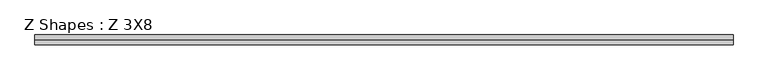
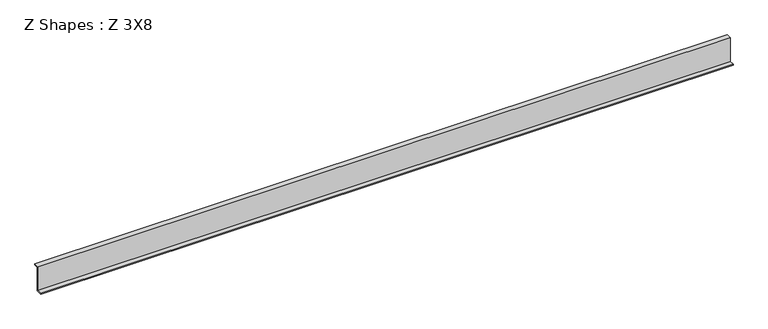
"""IFC4 building model written with IfcOpenShell, lengths in millimetres: beam geometry, Z Shapes : Z 3X8."""

from ifc_helpers import new_model, si_unit, frame, origin, place, context, project, spatial, polyline, outline, extrude, source, transform, mapped, element, save


def z_shapes_z_3x8_3d6c6c97(model_context):
    return source(origin(), model_context, "Body", "SweptSolid", [
        extrude(outline(polyline([(57.2805719, 92.452825), (27.1991352, 92.452825), (27.1991352, -98.809175), (-18.9194281, -98.809175), (-18.9194281, -92.459175), (19.1805719, -92.459175), (19.1805719, 102.104825), (57.2805719, 102.104825), (57.2805719, 92.452825)])), frame((-2667.0, 0.0, 0.0), z_axis=(1.0, 0.0, 0.0), x_axis=(0.0, 1.0, 0.0)), (0.0, 0.0, 1.0), 5334.0),
    ])


if __name__ == "__main__":
    model = new_model("IFC4")
    model_context = context("Model", 3, world=origin())
    ifc_project = project(units=[si_unit("LENGTHUNIT", "METRE", prefix="MILLI")], contexts=[model_context])
    site = spatial("IfcSite", under=ifc_project)
    building = spatial("IfcBuilding", under=site)
    placement = place(None, origin())
    z_shapes_z_3x8_shape = z_shapes_z_3x8_3d6c6c97(model_context)
    element("IfcBeam", 1, ObjectType="Z Shapes : Z 3X8", at=placement, inside=building, context=model_context, shape_type="MappedRepresentation", body=[
        mapped(z_shapes_z_3x8_shape, transform((0.0, 0.0, 0.0), x_axis=(1.0, 0.0, 0.0), y_axis=(0.0, 1.0, 0.0), z_axis=(0.0, 0.0, 1.0))),
    ])
    save(model, "model.ifc")

# Revit data of these elements
# Type "Z Shapes : Z 3X8"
#   Section Name Key = "W12x26"
#   Assembly Code = "B10"
#   Width = 76.2 mm
#   Web Thickness = 5.842 mm
#   Web Fillet = 7.62 mm
#   Warping Constant = 163001.3 cm⁶
#   Torsional Moment of Inertia = 12.4869 cm⁴
#   Section Area = 7.65 in²
#   Plastic Modulus weak axis = 0.00472801 (stored number, unit not read)
#   Plastic Modulus strong axis = 0.0215278 (stored number, unit not read)
#   Perimeter = 15.0571 m²/m
#   Nominal Weight = 379.441 N/m
#   Moment of Inertia weak axis = 720.08 cm⁴
#   Moment of Inertia strong axis = 8491.12 cm⁴
#   Height = 184.912 mm
#   Flange Thickness = 9.652 mm
#   Elastic Modulus weak axis = 0.00309028 (stored number, unit not read)
#   Elastic Modulus strong axis = 0.0193287 (stored number, unit not read)
#   Centroid Vertical = 92.456 mm
#   Centroid Horizontal = 38.1 mm
#   Length [instance default] = 5' - 0"
#   Structural Material [instance default] = Steel ASTM A992
#   Principal Axes Angle = 0
# Element 1 (IfcBeam, "Z Shapes : Z 3X8")
#   Structural Material = accent 2
#   Materials on its faces: "accent 2"
# Materials
#   "Steel ASTM A992": class "Metal", colour RGB 189 187 185, transparency 0, Description = "Structural steel 50ksi", Cost = 0
#   "accent 2": class "Wood", colour RGB 80 80 80, transparency 0, Description = "Wood framing, thermal airspace", Cost = 0
